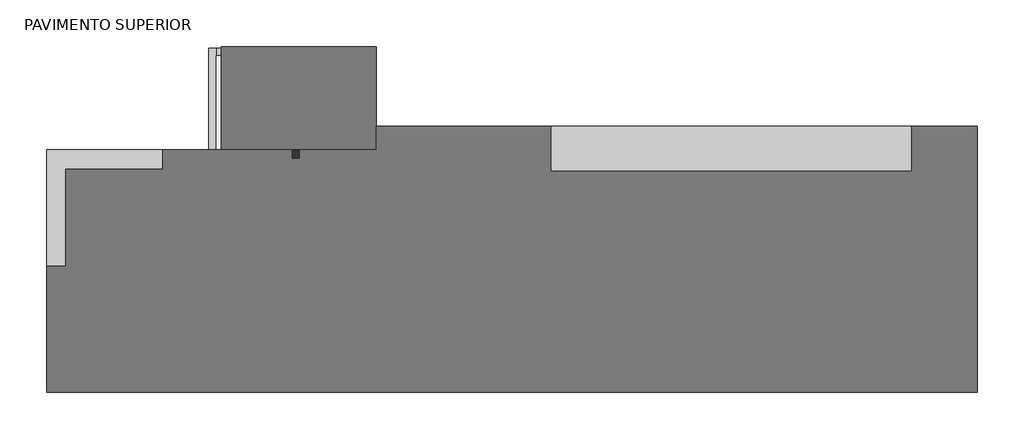
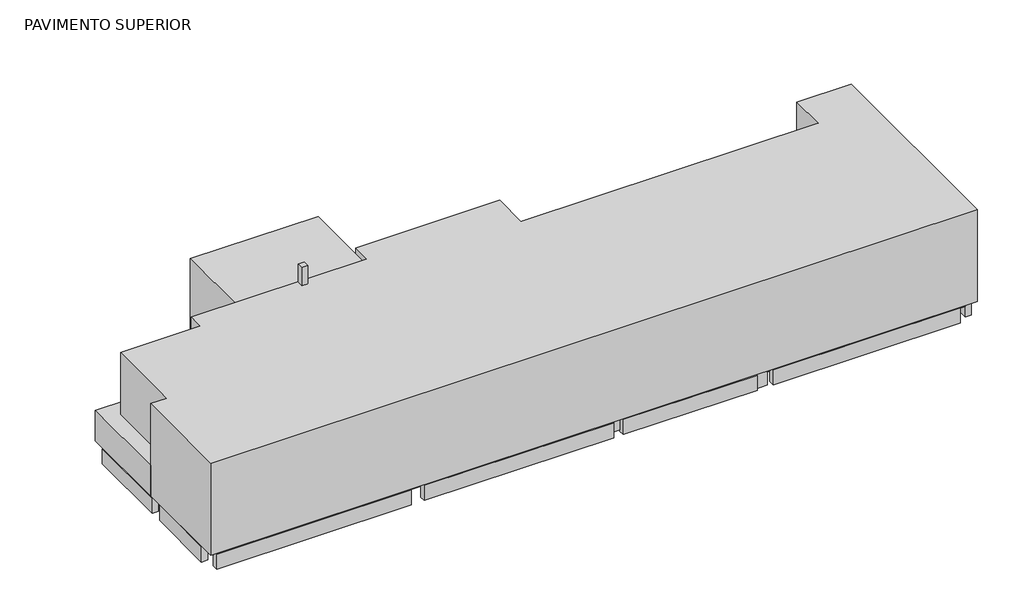
# One storey: 21 beams, 14 slabs, 2 proxies, 1 column.
# Revit data of these elements (continued)
# Element 11 (IfcBeam, "TQS - Viga retangular : 19.0 x 50.0") (continued)
#   Resultado de Ensaios fck (MPa) = 0
#   Unique TQS ID = -269
#   Principal = yes
#   Structural Material = none
#   Phase Created = CC_AP/ESTR
# Element 12 (IfcBeam, "TQS - Viga retangular : 19.0 x 50.0")
#   Uso = "ESTRUTURA"
#   Titulo = "V212"
#   Chave = "-271"
#   Tipo Elemento = "Viga"
#   SHA1 = "8138B3183DD0AFA166592BC9D25644F30CE3F0DB"
#   Revisão = ""
#   Tipo de carga = ""
#   Divisor de flexao = ""
#   Secao = ""
#   Configuracao = ""
#   Angulo (graus) = ""
#   Detalhamento = ""
#   Casos de vento manual = ""
#   Tipo = ""
#   Alcas = ""
#   Furos = ""
#   Pino = ""
#   Distribuicao = ""
#   Solidarizado = ""
#   Solidarizar na montagem = ""
#   Unir com o próximo = ""
#   Grupo pre moldado = ""
#   Verificado = ""
#   Concreto C = ""
#   Taxa de armadura (kgf/m³) = 0
#   Carga (tf/m²) = 0
#   Carga (tf/m) = 0
#   Carga (tf) = 0
#   Altura = 0.50 m
#   Rebaixo = 0.07 m
#   Largura = 0.19 m
#   Distancia a face = 0.00 m
#   Distancia ao eixo = 0.00 m
#   Altura gerber esquerda = 0.00 m
#   Largura gerber esquerda = 0.00 m
#   Altura gerber direita = 0.00 m
#   Largura gerber direita = 0.00 m
#   Resultado de Ensaios fck (MPa) = 0
#   Unique TQS ID = -271
#   Principal = yes
#   Structural Material = none
#   Phase Created = CC_AP/ESTR
# Element 13 (IfcBeam, "TQS - Viga retangular : 19.0 x 50.0")
#   Uso = "ESTRUTURA"
#   Titulo = "V204"
#   Chave = "-275"
#   Tipo Elemento = "Viga"
#   SHA1 = "02E3894711F00981ED511C33D176E4C517E4EA69"
#   Revisão = ""
#   Tipo de carga = ""
#   Divisor de flexao = ""
#   Secao = ""
#   Configuracao = ""
#   Angulo (graus) = ""
#   Detalhamento = ""
#   Casos de vento manual = ""
#   Tipo = ""
#   Alcas = ""
#   Furos = ""
#   Pino = ""
#   Distribuicao = ""
#   Solidarizado = ""
#   Solidarizar na montagem = ""
#   Unir com o próximo = ""
#   Grupo pre moldado = ""
#   Verificado = ""
#   Concreto C = ""
#   Taxa de armadura (kgf/m³) = 0
#   Carga (tf/m²) = 0
#   Carga (tf/m) = 0
#   Carga (tf) = 0
#   Altura = 0.50 m
#   Rebaixo = 0.07 m
#   Largura = 0.19 m
#   Distancia a face = 0.00 m
#   Distancia ao eixo = 0.00 m
#   Altura gerber esquerda = 0.00 m
#   Largura gerber esquerda = 0.00 m
#   Altura gerber direita = 0.00 m
#   Largura gerber direita = 0.00 m
#   Resultado de Ensaios fck (MPa) = 0
#   Unique TQS ID = -275
#   Principal = yes
#   Structural Material = none
#   Phase Created = CC_AP/ESTR
# Element 14 (IfcBeam, "TQS - Viga retangular : 19.0 x 50.0")
#   Uso = "ESTRUTURA"
#   Titulo = "V220"
#   Chave = "-277"
#   Tipo Elemento = "Viga"
#   SHA1 = "53FFBE44C6DCAED37B6C8CE186A7B735EF97D81B"
#   Revisão = ""
#   Tipo de carga = ""
#   Divisor de flexao = ""
#   Secao = ""
#   Configuracao = ""
#   Angulo (graus) = ""
#   Detalhamento = ""
#   Casos de vento manual = ""
#   Tipo = ""
#   Alcas = ""
#   Furos = ""
#   Pino = ""
#   Distribuicao = ""
#   Solidarizado = ""
#   Solidarizar na montagem = ""
#   Unir com o próximo = ""
#   Grupo pre moldado = ""
#   Verificado = ""
#   Concreto C = ""
#   Taxa de armadura (kgf/m³) = 0
#   Carga (tf/m²) = 0
#   Carga (tf/m) = 0
#   Carga (tf) = 0
#   Altura = 0.50 m
#   Rebaixo = 0.07 m
#   Largura = 0.19 m
#   Distancia a face = 0.00 m
#   Distancia ao eixo = 0.00 m
#   Altura gerber esquerda = 0.00 m
#   Largura gerber esquerda = 0.00 m
#   Altura gerber direita = 0.00 m
#   Largura gerber direita = 0.00 m
#   Resultado de Ensaios fck (MPa) = 0
#   Unique TQS ID = -277
#   Principal = yes
#   Structural Material = none
#   Phase Created = CC_AP/ESTR
# Element 15 (IfcBeam, "TQS - Viga retangular : 19.0 x 50.0")
#   Uso = "ESTRUTURA"
#   Titulo = "V205"
#   Chave = "-282"
#   Tipo Elemento = "Viga"
#   SHA1 = "42659F1FB713DA20C0E97ED290CCDAD82A2232BE"
#   Revisão = ""
#   Tipo de carga = ""
#   Divisor de flexao = ""
#   Secao = ""
#   Configuracao = ""
#   Angulo (graus) = ""
#   Detalhamento = ""
#   Casos de vento manual = ""
#   Tipo = ""
#   Alcas = ""
#   Furos = ""
#   Pino = ""
#   Distribuicao = ""
#   Solidarizado = ""
#   Solidarizar na montagem = ""
#   Unir com o próximo = ""
#   Grupo pre moldado = ""
#   Verificado = ""
#   Concreto C = ""
#   Taxa de armadura (kgf/m³) = 0
#   Carga (tf/m²) = 0
#   Carga (tf/m) = 0
#   Carga (tf) = 0
#   Altura = 0.50 m
#   Rebaixo = 0.07 m
#   Largura = 0.19 m
#   Distancia a face = 0.00 m
#   Distancia ao eixo = 0.00 m
#   Altura gerber esquerda = 0.00 m
#   Largura gerber esquerda = 0.00 m
#   Altura gerber direita = 0.00 m
#   Largura gerber direita = 0.00 m
#   Resultado de Ensaios fck (MPa) = 0
#   Unique TQS ID = -282
#   Principal = yes
#   Structural Material = none
#   Phase Created = CC_AP/ESTR
# Element 16 (IfcBeam, "TQS - Viga retangular : 19.0 x 50.0")
#   Uso = "ESTRUTURA"
#   Titulo = "V213"
#   Chave = "-292"
#   Tipo Elemento = "Viga"
#   SHA1 = "0FE3684D1E2234CA12F99F83675A4BD65DC506E8"
#   Revisão = ""
#   Tipo de carga = ""
#   Divisor de flexao = ""
#   Secao = ""
#   Configuracao = ""
#   Angulo (graus) = ""
#   Detalhamento = ""
#   Casos de vento manual = ""
#   Tipo = ""
#   Alcas = ""
#   Furos = ""
#   Pino = ""
#   Distribuicao = ""
#   Solidarizado = ""
#   Solidarizar na montagem = ""
#   Unir com o próximo = ""
#   Grupo pre moldado = ""
#   Verificado = ""
#   Concreto C = ""
#   Taxa de armadura (kgf/m³) = 0
#   Carga (tf/m²) = 0
#   Carga (tf/m) = 0
#   Carga (tf) = 0
#   Altura = 0.50 m
#   Rebaixo = 0.07 m
#   Largura = 0.19 m
#   Distancia a face = 0.00 m
#   Distancia ao eixo = 0.00 m
#   Altura gerber esquerda = 0.00 m
#   Largura gerber esquerda = 0.00 m
#   Altura gerber direita = 0.00 m
#   Largura gerber direita = 0.00 m
#   Resultado de Ensaios fck (MPa) = 0
#   Unique TQS ID = -292
#   Principal = yes
#   Structural Material = none
#   Phase Created = CC_AP/ESTR
# Element 17 (IfcBeam, "TQS - Viga retangular : 19.0 x 50.0")
#   Uso = "ESTRUTURA"
#   Titulo = "V216"
#   Chave = "-293"
#   Tipo Elemento = "Viga"
#   SHA1 = "A379C6197F25C7CB47ACBD41020AB1BAF3A8190D"
#   Revisão = ""
#   Tipo de carga = ""
#   Divisor de flexao = ""
#   Secao = ""
#   Configuracao = ""
#   Angulo (graus) = ""
#   Detalhamento = ""
#   Casos de vento manual = ""
#   Tipo = ""
#   Alcas = ""
#   Furos = ""
#   Pino = ""
#   Distribuicao = ""
#   Solidarizado = ""
#   Solidarizar na montagem = ""
#   Unir com o próximo = ""
#   Grupo pre moldado = ""
#   Verificado = ""
#   Concreto C = ""
#   Taxa de armadura (kgf/m³) = 0
#   Carga (tf/m²) = 0
#   Carga (tf/m) = 0
#   Carga (tf) = 0
#   Altura = 0.50 m
#   Rebaixo = 0.07 m
#   Largura = 0.19 m
#   Distancia a face = 0.00 m
#   Distancia ao eixo = 0.00 m
#   Altura gerber esquerda = 0.00 m
#   Largura gerber esquerda = 0.00 m
#   Altura gerber direita = 0.00 m
#   Largura gerber direita = 0.00 m
#   Resultado de Ensaios fck (MPa) = 0
#   Unique TQS ID = -293
#   Principal = yes
#   Structural Material = none
#   Phase Created = CC_AP/ESTR
# Element 18 (IfcBeam, "TQS - Viga retangular : 19.0 x 50.0")
#   Uso = "ESTRUTURA"
#   Titulo = "V201"
#   Chave = "-294"
#   Tipo Elemento = "Viga"
#   SHA1 = "3FA94C587EE4F3BD96CF329630B49136817C541B"
#   Revisão = ""
#   Tipo de carga = ""
#   Divisor de flexao = ""
#   Secao = ""
#   Configuracao = ""
#   Angulo (graus) = ""
#   Detalhamento = ""
#   Casos de vento manual = ""
#   Tipo = ""
#   Alcas = ""
#   Furos = ""
#   Pino = ""
#   Distribuicao = ""
#   Solidarizado = ""
#   Solidarizar na montagem = ""
#   Unir com o próximo = ""
#   Grupo pre moldado = ""
#   Verificado = ""
#   Concreto C = ""
#   Taxa de armadura (kgf/m³) = 0
#   Carga (tf/m²) = 0
#   Carga (tf/m) = 0
#   Carga (tf) = 0
#   Altura = 0.50 m
#   Rebaixo = 0.07 m
#   Largura = 0.19 m
#   Distancia a face = 0.00 m
#   Distancia ao eixo = 0.00 m
#   Altura gerber esquerda = 0.00 m
#   Largura gerber esquerda = 0.00 m
#   Altura gerber direita = 0.00 m
#   Largura gerber direita = 0.00 m
#   Resultado de Ensaios fck (MPa) = 0
#   Unique TQS ID = -294
#   Principal = yes
#   Structural Material = none
#   Phase Created = CC_AP/ESTR
# Element 19 (IfcBeam, "TQS - Viga retangular : 19.0 x 50.0")
#   Uso = "ESTRUTURA"
#   Titulo = "V203"
#   Chave = "-1337"
#   Tipo Elemento = "Viga"
#   SHA1 = "F25A04961C3A0A77CFDF86D87ECBEE6AEAF2B145"
#   Revisão = ""
#   Tipo de carga = ""
#   Divisor de flexao = ""
#   Secao = ""
#   Configuracao = ""
#   Angulo (graus) = ""
#   Detalhamento = ""
#   Casos de vento manual = ""
#   Tipo = ""
#   Alcas = ""
#   Furos = ""
#   Pino = ""
#   Distribuicao = ""
#   Solidarizado = ""
#   Solidarizar na montagem = ""
#   Unir com o próximo = ""
#   Grupo pre moldado = ""
#   Verificado = ""
#   Concreto C = ""
#   Taxa de armadura (kgf/m³) = 0
#   Carga (tf/m²) = 0
#   Carga (tf/m) = 0
#   Carga (tf) = 0
#   Altura = 0.50 m
#   Rebaixo = 0.07 m
#   Largura = 0.19 m
#   Distancia a face = 0.00 m
#   Distancia ao eixo = 0.00 m
#   Altura gerber esquerda = 0.00 m
#   Largura gerber esquerda = 0.00 m
#   Altura gerber direita = 0.00 m
#   Largura gerber direita = 0.00 m
#   Resultado de Ensaios fck (MPa) = 0
#   Unique TQS ID = -1337
#   Principal = yes
#   Structural Material = none
#   Phase Created = CC_AP/ESTR
# Element 20 (IfcBeam, "TQS - Viga retangular : 35.0 x 50.0")
#   Uso = "ESTRUTURA"
#   Titulo = "V218"
#   Chave = "-1330"
#   Tipo Elemento = "Viga"
#   SHA1 = "DF59D9C5ECE1DAFADA315DD633BF351C28CD7B23"
#   Revisão = ""
#   Tipo de carga = ""
#   Divisor de flexao = ""
#   Secao = ""
#   Configuracao = ""
#   Angulo (graus) = ""
#   Detalhamento = ""
#   Casos de vento manual = ""
#   Tipo = ""
#   Alcas = ""
#   Furos = ""
#   Pino = ""
#   Distribuicao = ""
#   Solidarizado = ""
#   Solidarizar na montagem = ""
#   Unir com o próximo = ""
#   Grupo pre moldado = ""
#   Verificado = ""
#   Concreto C = ""
#   Taxa de armadura (kgf/m³) = 0
#   Carga (tf/m²) = 0
#   Carga (tf/m) = 0
#   Carga (tf) = 0
#   Altura = 0.50 m
#   Rebaixo = 0.16 m
#   Largura = 0.35 m
#   Distancia a face = 0.00 m
#   Distancia ao eixo = 0.00 m
#   Altura gerber esquerda = 0.00 m
#   Largura gerber esquerda = 0.00 m
#   Altura gerber direita = 0.00 m
#   Largura gerber direita = 0.00 m
#   Resultado de Ensaios fck (MPa) = 0
#   Unique TQS ID = -1330
#   Principal = yes
#   Structural Material = none
#   Phase Created = CC_AP/ESTR
# Element 21 (IfcBeam, "TQS - Viga retangular : 35.0 x 59.0")
#   Uso = "ESTRUTURA"
#   Titulo = "V218"
#   Chave = "-1329"
#   Tipo Elemento = "Viga"
#   SHA1 = "67D04BBC0D1EFB8924A6F9E6F0DB65A2FA8FB170"
#   Revisão = ""
#   Tipo de carga = ""
#   Divisor de flexao = ""
#   Secao = ""
#   Configuracao = ""
#   Angulo (graus) = ""
#   Detalhamento = ""
#   Casos de vento manual = ""
#   Tipo = ""
#   Alcas = ""
#   Furos = ""
#   Pino = ""
#   Distribuicao = ""
#   Solidarizado = ""
#   Solidarizar na montagem = ""
#   Unir com o próximo = ""
#   Grupo pre moldado = ""
#   Verificado = ""
#   Concreto C = ""
#   Taxa de armadura (kgf/m³) = 0
#   Carga (tf/m²) = 0
#   Carga (tf/m) = 0
#   Carga (tf) = 0
#   Altura = 0.59 m
#   Rebaixo = 0.07 m
#   Largura = 0.35 m
#   Distancia a face = 0.00 m
#   Distancia ao eixo = 0.00 m
#   Altura gerber esquerda = 0.00 m
#   Largura gerber esquerda = 0.00 m
#   Altura gerber direita = 0.00 m
#   Largura gerber direita = 0.00 m
#   Resultado de Ensaios fck (MPa) = 0
#   Unique TQS ID = -1329
#   Principal = yes
#   Structural Material = none
#   Phase Created = CC_AP/ESTR
# Element 22 (IfcBuildingElementProxy, "SUÍTES E SALA ÍNTIMA : SUÍTES E SALA ÍNTIMA")
#   Phase Created = CC_EV
#   Materials on its faces: "Forma padrão"
# Element 23 (IfcBuildingElementProxy, "TERRAÇO : TERRAÇO")
#   Phase Created = CC_EV
#   Materials on its faces: "Forma padrão"
# Element 24 (IfcColumn, "TQS - Pilar retangular : 19.0 x 19.0")
#   Uso = "ESTRUTURA"
#   Titulo = "P17.2"
#   Chave = "P17.2//0"
#   Tipo Elemento = "Pilar"
#   SHA1 = "5EAE41CEDCF7AC730D71745C540256BEBFE0F897"
#   Revisão = ""
#   Tipo de carga = ""
#   Divisor de flexao = ""
#   Secao = "R 19/19 180°"
#   Configuracao = ""
#   Angulo (graus) = ""
#   Detalhamento = ""
#   Casos de vento manual = ""
#   Tipo = ""
#   Alcas = ""
#   Furos = ""
#   Pino = ""
#   Distribuicao = ""
#   Solidarizado = ""
#   Solidarizar na montagem = ""
#   Unir com o próximo = ""
#   Grupo pre moldado = ""
#   Verificado = ""
#   Concreto C = ""
#   Taxa de armadura (kgf/m³) = 0
#   Carga (tf/m²) = 0
#   Carga (tf/m) = 0
#   Carga (tf) = 0
#   Altura = 3.05 m
#   Rebaixo = 0.00 m
#   Altura da fundacao = 0.00 m
#   Largura = 0.00 m
#   Distancia a face = 0.00 m
#   Distancia ao eixo = 0.00 m
#   Resultado de Ensaios fck (MPa) = 0
#   Unique TQS ID = -1881
#   Principal = yes
#   Nasce = yes
#   Morre = yes
#   Cabeca de Pilar = no
#   Structural Material = Concrete - Cast-in-Place Concrete
#   Phase Created = CC_AP/ESTR
#   Materials on its faces: "Concrete - Cast-in-Place Concrete"
# Element 25 (IfcSlab, "TQS h=15")
#   Uso = "ESTRUTURA"
#   Titulo = "L2"
#   Chave = "-293"
#   Tipo Elemento = "Laje"
#   SHA1 = "30CE78691B5EE77FC65FFF8CB4530939F77CBC39"
#   Revisão = ""
#   Tipo de carga = ""
#   Divisor de flexao = ""
#   Fabricante = ""
#   Enchimento = ""
#   Mini painel = ""
#   Blocos por nervura = ""
#   Secao = ""
#   Configuracao = ""
#   Angulo (graus) = "0"
#   Detalhamento = ""
#   Casos de vento manual = ""
#   Tipo = "Pré-moldada"
#   Alcas = ""
#   Furos = ""
#   Pino = ""
#   Distribuicao = ""
#   Solidarizado = ""
#   Solidarizar na montagem = ""
#   Unir com o próximo = ""
#   Grupo pre moldado = ""
#   Verificado = ""
#   Concreto C = ""
#   Height Offset From Level = -0.07 m
#   Taxa de armadura (kgf/m³) = 0
#   Carga (tf/m²) = 0
#   Carga (tf/m) = 0
#   Carga (tf) = 0
#   Altura = 0.15 m
#   Capa = 0.04 m
#   Capa inferior = 0.00 m
#   Altura da nervura = 0.11 m
#   Enchimento (tf/m³) = 0.02
#   Largura inferior X = 0.00 m
#   Distancia inferior X = 0.00 m
#   Largura inferior Y = 0.00 m
#   Distancia inferior Y = 0.00 m
#   Largura vigota = 0.00 m
#   Altura vigota = 0.00 m
#   Largura perfil = 0.00 m
#   Largura aba = 0.00 m
#   Altura perfil = 0.00 m
#   Nervura secundaria = 0.00 m
#   Desconto nervura secundaria = 0.00 m
#   Rebaixo = -0.07 m
#   Largura = 0.00 m
#   Distancia a face = 0.00 m
#   Distancia ao eixo = 0.00 m
#   Resultado de Ensaios fck (MPa) = 0
#   built-in parameter 1001954 = 1
#   Unique TQS ID = -293
#   Principal = yes
#   Phase Created = CC_AP/ESTR
#   Materials on its faces: ".MATERIAL GENÉRICO LAJE E PISO"
# Element 26 (IfcSlab, "TQS h=15")
#   Uso = "ESTRUTURA"
#   Titulo = "L8"
#   Chave = "-294"
#   Tipo Elemento = "Laje"
#   SHA1 = "A0E1DD69F653FC0ADE227BB067D3F3136C230378"
#   Revisão = ""
#   Tipo de carga = ""
#   Divisor de flexao = ""
#   Fabricante = ""
#   Enchimento = ""
#   Mini painel = ""
#   Blocos por nervura = ""
#   Secao = ""
#   Configuracao = ""
#   Angulo (graus) = "0"
#   Detalhamento = ""
#   Casos de vento manual = ""
#   Tipo = "Pré-moldada"
#   Alcas = ""
#   Furos = ""
#   Pino = ""
#   Distribuicao = ""
#   Solidarizado = ""
#   Solidarizar na montagem = ""
#   Unir com o próximo = ""
#   Grupo pre moldado = ""
#   Verificado = ""
#   Concreto C = ""
#   Height Offset From Level = -0.07 m
#   Taxa de armadura (kgf/m³) = 0
#   Carga (tf/m²) = 0
#   Carga (tf/m) = 0
#   Carga (tf) = 0
#   Altura = 0.15 m
#   Capa = 0.04 m
#   Capa inferior = 0.00 m
#   Altura da nervura = 0.11 m
#   Enchimento (tf/m³) = 0.02
#   Largura inferior X = 0.00 m
#   Distancia inferior X = 0.00 m
#   Largura inferior Y = 0.00 m
#   Distancia inferior Y = 0.00 m
#   Largura vigota = 0.00 m
#   Altura vigota = 0.00 m
#   Largura perfil = 0.00 m
#   Largura aba = 0.00 m
#   Altura perfil = 0.00 m
#   Nervura secundaria = 0.00 m
#   Desconto nervura secundaria = 0.00 m
#   Rebaixo = -0.07 m
#   Largura = 0.00 m
#   Distancia a face = 0.00 m
#   Distancia ao eixo = 0.00 m
#   Resultado de Ensaios fck (MPa) = 0
#   built-in parameter 1001954 = 1
#   Unique TQS ID = -294
#   Principal = yes
#   Phase Created = CC_AP/ESTR
#   Materials on its faces: ".MATERIAL GENÉRICO LAJE E PISO"
# Element 27 (IfcSlab, "TQS h=15")
#   Uso = "ESTRUTURA"
#   Titulo = "L12"
#   Chave = "-1341"
#   Tipo Elemento = "Laje"
#   SHA1 = "62DBD7FB482137E78B4EBE55A5ED8AF7F76A63B1"
#   Revisão = ""
#   Tipo de carga = ""
#   Divisor de flexao = ""
#   Fabricante = ""
#   Enchimento = ""
#   Mini painel = ""
#   Blocos por nervura = ""
#   Secao = ""
#   Configuracao = ""
#   Angulo (graus) = "90"
#   Detalhamento = ""
#   Casos de vento manual = ""
#   Tipo = "Pré-moldada"
#   Alcas = ""
#   Furos = ""
#   Pino = ""
#   Distribuicao = ""
#   Solidarizado = ""
#   Solidarizar na montagem = ""
#   Unir com o próximo = ""
#   Grupo pre moldado = ""
#   Verificado = ""
#   Concreto C = ""
#   Height Offset From Level = -0.07 m
#   Taxa de armadura (kgf/m³) = 0
#   Carga (tf/m²) = 0
#   Carga (tf/m) = 0
#   Carga (tf) = 0
#   Altura = 0.15 m
#   Capa = 0.04 m
#   Capa inferior = 0.00 m
#   Altura da nervura = 0.11 m
#   Enchimento (tf/m³) = 0.02
#   Largura inferior X = 0.00 m
#   Distancia inferior X = 0.00 m
#   Largura inferior Y = 0.00 m
#   Distancia inferior Y = 0.00 m
#   Largura vigota = 0.00 m
#   Altura vigota = 0.00 m
#   Largura perfil = 0.00 m
#   Largura aba = 0.00 m
#   Altura perfil = 0.00 m
#   Nervura secundaria = 0.00 m
#   Desconto nervura secundaria = 0.00 m
#   Rebaixo = -0.07 m
#   Largura = 0.00 m
#   Distancia a face = 0.00 m
#   Distancia ao eixo = 0.00 m
#   Resultado de Ensaios fck (MPa) = 0
#   built-in parameter 1001954 = 1
#   Unique TQS ID = -1341
#   Principal = yes
#   Phase Created = CC_AP/ESTR
#   Materials on its faces: ".MATERIAL GENÉRICO LAJE E PISO"
# Element 28 (IfcSlab, "TQS h=15")
#   Uso = "ESTRUTURA"
#   Titulo = "L7"
#   Chave = "-289"
#   Tipo Elemento = "Laje"
#   SHA1 = "00FB641EB890BE101A5F35BC568EFA8C03036441"
#   Revisão = ""
#   Tipo de carga = ""
#   Divisor de flexao = ""
#   Fabricante = ""
#   Enchimento = ""
#   Mini painel = ""
#   Blocos por nervura = ""
#   Secao = ""
#   Configuracao = ""
#   Angulo (graus) = "90"
#   Detalhamento = ""
#   Casos de vento manual = ""
#   Tipo = "Pré-moldada"
#   Alcas = ""
#   Furos = ""
#   Pino = ""
#   Distribuicao = ""
#   Solidarizado = ""
#   Solidarizar na montagem = ""
#   Unir com o próximo = ""
#   Grupo pre moldado = ""
#   Verificado = ""
#   Concreto C = ""
#   Height Offset From Level = -0.07 m
#   Taxa de armadura (kgf/m³) = 0
#   Carga (tf/m²) = 0
#   Carga (tf/m) = 0
#   Carga (tf) = 0
#   Altura = 0.15 m
#   Capa = 0.04 m
#   Capa inferior = 0.00 m
#   Altura da nervura = 0.11 m
#   Enchimento (tf/m³) = 0.02
#   Largura inferior X = 0.00 m
#   Distancia inferior X = 0.00 m
#   Largura inferior Y = 0.00 m
#   Distancia inferior Y = 0.00 m
#   Largura vigota = 0.00 m
#   Altura vigota = 0.00 m
#   Largura perfil = 0.00 m
#   Largura aba = 0.00 m
#   Altura perfil = 0.00 m
#   Nervura secundaria = 0.00 m
#   Desconto nervura secundaria = 0.00 m
#   Rebaixo = -0.07 m
#   Largura = 0.00 m
#   Distancia a face = 0.00 m
#   Distancia ao eixo = 0.00 m
#   Resultado de Ensaios fck (MPa) = 0
#   built-in parameter 1001954 = 1
#   Unique TQS ID = -289
#   Principal = yes
#   Phase Created = CC_AP/ESTR
#   Materials on its faces: ".MATERIAL GENÉRICO LAJE E PISO"
# Element 29 (IfcSlab, "TQS h=15")
#   Uso = "ESTRUTURA"
#   Titulo = "L3"
#   Chave = "-290"
#   Tipo Elemento = "Laje"
#   SHA1 = "5CC856C49E54B4625D4D3CA5C635EB29D7F82A16"
#   Revisão = ""
#   Tipo de carga = ""
#   Divisor de flexao = ""
#   Fabricante = ""
#   Enchimento = ""
#   Mini painel = ""
#   Blocos por nervura = ""
#   Secao = ""
#   Configuracao = ""
#   Angulo (graus) = "90"
#   Detalhamento = ""
#   Casos de vento manual = ""
#   Tipo = "Pré-moldada"
#   Alcas = ""
#   Furos = ""
#   Pino = ""
#   Distribuicao = ""
#   Solidarizado = ""
#   Solidarizar na montagem = ""
#   Unir com o próximo = ""
#   Grupo pre moldado = ""
#   Verificado = ""
#   Concreto C = ""
#   Height Offset From Level = -0.07 m
#   Taxa de armadura (kgf/m³) = 0
#   Carga (tf/m²) = 0
#   Carga (tf/m) = 0
#   Carga (tf) = 0
#   Altura = 0.15 m
#   Capa = 0.04 m
#   Capa inferior = 0.00 m
#   Altura da nervura = 0.11 m
#   Enchimento (tf/m³) = 0.02
#   Largura inferior X = 0.00 m
#   Distancia inferior X = 0.00 m
#   Largura inferior Y = 0.00 m
#   Distancia inferior Y = 0.00 m
#   Largura vigota = 0.00 m
#   Altura vigota = 0.00 m
#   Largura perfil = 0.00 m
#   Largura aba = 0.00 m
#   Altura perfil = 0.00 m
#   Nervura secundaria = 0.00 m
#   Desconto nervura secundaria = 0.00 m
#   Rebaixo = -0.07 m
#   Largura = 0.00 m
#   Distancia a face = 0.00 m
#   Distancia ao eixo = 0.00 m
#   Resultado de Ensaios fck (MPa) = 0
#   built-in parameter 1001954 = 1
#   Unique TQS ID = -290
#   Principal = yes
#   Phase Created = CC_AP/ESTR
#   Materials on its faces: ".MATERIAL GENÉRICO LAJE E PISO"
# Element 30 (IfcSlab, "TQS h=15")
#   Uso = "ESTRUTURA"
#   Titulo = "L4"
#   Chave = "-291"
#   Tipo Elemento = "Laje"
#   SHA1 = "E1E752CC52417E869C2ECB3AAEF17918D9AB4584"
#   Revisão = ""
#   Tipo de carga = ""
#   Divisor de flexao = ""
#   Fabricante = ""
#   Enchimento = ""
#   Mini painel = ""
#   Blocos por nervura = ""
#   Secao = ""
#   Configuracao = ""
#   Angulo (graus) = "90"
#   Detalhamento = ""
#   Casos de vento manual = ""
#   Tipo = "Pré-moldada"
#   Alcas = ""
#   Furos = ""
#   Pino = ""
#   Distribuicao = ""
#   Solidarizado = ""
#   Solidarizar na montagem = ""
#   Unir com o próximo = ""
#   Grupo pre moldado = ""
#   Verificado = ""
#   Concreto C = ""
#   Height Offset From Level = -0.07 m
#   Taxa de armadura (kgf/m³) = 0
#   Carga (tf/m²) = 0
#   Carga (tf/m) = 0
#   Carga (tf) = 0
#   Altura = 0.15 m
#   Capa = 0.04 m
#   Capa inferior = 0.00 m
#   Altura da nervura = 0.11 m
#   Enchimento (tf/m³) = 0.02
#   Largura inferior X = 0.00 m
#   Distancia inferior X = 0.00 m
#   Largura inferior Y = 0.00 m
#   Distancia inferior Y = 0.00 m
#   Largura vigota = 0.00 m
#   Altura vigota = 0.00 m
#   Largura perfil = 0.00 m
#   Largura aba = 0.00 m
#   Altura perfil = 0.00 m
#   Nervura secundaria = 0.00 m
#   Desconto nervura secundaria = 0.00 m
#   Rebaixo = -0.07 m
#   Largura = 0.00 m
#   Distancia a face = 0.00 m
#   Distancia ao eixo = 0.00 m
#   Resultado de Ensaios fck (MPa) = 0
#   built-in parameter 1001954 = 1
#   Unique TQS ID = -291
#   Principal = yes
#   Phase Created = CC_AP/ESTR
#   Materials on its faces: ".MATERIAL GENÉRICO LAJE E PISO"
# Element 31 (IfcSlab, "TQS h=15")
#   Uso = "ESTRUTURA"
#   Titulo = "L1"
#   Chave = "-782"
#   Tipo Elemento = "Laje"
#   SHA1 = "243054E1496AE50C7A59F49C35E9A6C4CBFBF802"
#   Revisão = ""
#   Tipo de carga = ""
#   Divisor de flexao = ""
#   Fabricante = ""
#   Enchimento = ""
#   Mini painel = ""
#   Blocos por nervura = ""
#   Secao = ""
#   Configuracao = ""
#   Angulo (graus) = "0"
#   Detalhamento = ""
#   Casos de vento manual = ""
#   Tipo = "Pré-moldada"
#   Alcas = ""
#   Furos = ""
#   Pino = ""
#   Distribuicao = ""
#   Solidarizado = ""
#   Solidarizar na montagem = ""
#   Unir com o próximo = ""
#   Grupo pre moldado = ""
#   Verificado = ""
#   Concreto C = ""
#   Height Offset From Level = -0.07 m
#   Taxa de armadura (kgf/m³) = 0
#   Carga (tf/m²) = 0
#   Carga (tf/m) = 0
#   Carga (tf) = 0
#   Altura = 0.15 m
#   Capa = 0.04 m
#   Capa inferior = 0.00 m
#   Altura da nervura = 0.11 m
#   Enchimento (tf/m³) = 0.02
#   Largura inferior X = 0.00 m
#   Distancia inferior X = 0.00 m
#   Largura inferior Y = 0.00 m
#   Distancia inferior Y = 0.00 m
#   Largura vigota = 0.00 m
#   Altura vigota = 0.00 m
#   Largura perfil = 0.00 m
#   Largura aba = 0.00 m
#   Altura perfil = 0.00 m
#   Nervura secundaria = 0.00 m
#   Desconto nervura secundaria = 0.00 m
#   Rebaixo = -0.07 m
#   Largura = 0.00 m
#   Distancia a face = 0.00 m
#   Distancia ao eixo = 0.00 m
#   Resultado de Ensaios fck (MPa) = 0
#   built-in parameter 1001954 = 1
#   Unique TQS ID = -782
#   Principal = yes
#   Phase Created = CC_AP/ESTR
#   Materials on its faces: ".MATERIAL GENÉRICO LAJE E PISO"
# Element 32 (IfcSlab, "TQS h=15")
#   Uso = "ESTRUTURA"
#   Titulo = "L5"
#   Chave = "-324"
#   Tipo Elemento = "Laje"
#   SHA1 = "6BEC4C6D90655AA68C15FC8554BD79BC3B34892D"
#   Revisão = ""
#   Tipo de carga = ""
#   Divisor de flexao = ""
#   Fabricante = ""
#   Enchimento = ""
#   Mini painel = ""
#   Blocos por nervura = ""
#   Secao = ""
#   Configuracao = ""
#   Angulo (graus) = "0"
#   Detalhamento = ""
#   Casos de vento manual = ""
#   Tipo = "Maciça"
#   Alcas = ""
#   Furos = ""
#   Pino = ""
#   Distribuicao = ""
#   Solidarizado = ""
#   Solidarizar na montagem = ""
#   Unir com o próximo = ""
#   Grupo pre moldado = ""
#   Verificado = ""
#   Concreto C = ""
#   Height Offset From Level = -0.07 m
#   Taxa de armadura (kgf/m³) = 0
#   Carga (tf/m²) = 0
#   Carga (tf/m) = 0
#   Carga (tf) = 0
#   Altura = 0.15 m
#   Capa = 0.00 m
#   Capa inferior = 0.00 m
#   Altura da nervura = 0.00 m
#   Enchimento (tf/m³) = 0
#   Largura inferior X = 0.00 m
#   Distancia inferior X = 0.00 m
#   Largura inferior Y = 0.00 m
#   Distancia inferior Y = 0.00 m
#   Largura vigota = 0.00 m
#   Altura vigota = 0.00 m
#   Largura perfil = 0.00 m
#   Largura aba = 0.00 m
#   Altura perfil = 0.00 m
#   Nervura secundaria = 0.00 m
#   Desconto nervura secundaria = 0.00 m
#   Rebaixo = -0.07 m
#   Largura = 0.00 m
#   Distancia a face = 0.00 m
#   Distancia ao eixo = 0.00 m
#   Resultado de Ensaios fck (MPa) = 0
#   built-in parameter 1001954 = 1
#   Unique TQS ID = -324
#   Principal = yes
#   Phase Created = CC_AP/ESTR
#   Materials on its faces: ".MATERIAL GENÉRICO LAJE E PISO"
# Element 33 (IfcSlab, "TQS h=15")
#   Uso = "ESTRUTURA"
#   Titulo = "L6"
#   Chave = "-325"
#   Tipo Elemento = "Laje"
#   SHA1 = "45A1BB14EB53BA680F766E33394AE66BA68CD49B"
#   Revisão = ""
#   Tipo de carga = ""
#   Divisor de flexao = ""
#   Fabricante = ""
#   Enchimento = ""
#   Mini painel = ""
#   Blocos por nervura = ""
#   Secao = ""
#   Configuracao = ""
#   Angulo (graus) = "0"
#   Detalhamento = ""
#   Casos de vento manual = ""
#   Tipo = "Maciça"
#   Alcas = ""
#   Furos = ""
#   Pino = ""
#   Distribuicao = ""
#   Solidarizado = ""
#   Solidarizar na montagem = ""
#   Unir com o próximo = ""
#   Grupo pre moldado = ""
#   Verificado = ""
#   Concreto C = ""
#   Height Offset From Level = -0.07 m
#   Taxa de armadura (kgf/m³) = 0
#   Carga (tf/m²) = 0
#   Carga (tf/m) = 0
#   Carga (tf) = 0
#   Altura = 0.15 m
#   Capa = 0.00 m
#   Capa inferior = 0.00 m
#   Altura da nervura = 0.00 m
#   Enchimento (tf/m³) = 0
#   Largura inferior X = 0.00 m
#   Distancia inferior X = 0.00 m
#   Largura inferior Y = 0.00 m
#   Distancia inferior Y = 0.00 m
#   Largura vigota = 0.00 m
#   Altura vigota = 0.00 m
#   Largura perfil = 0.00 m
#   Largura aba = 0.00 m
#   Altura perfil = 0.00 m
#   Nervura secundaria = 0.00 m
#   Desconto nervura secundaria = 0.00 m
#   Rebaixo = -0.07 m
#   Largura = 0.00 m
#   Distancia a face = 0.00 m
#   Distancia ao eixo = 0.00 m
#   Resultado de Ensaios fck (MPa) = 0
#   built-in parameter 1001954 = 1
#   Unique TQS ID = -325
#   Principal = yes
#   Phase Created = CC_AP/ESTR
#   Materials on its faces: ".MATERIAL GENÉRICO LAJE E PISO"
# Element 34 (IfcSlab, "TQS h=15")
#   Uso = "ESTRUTURA"
#   Titulo = "L10"
#   Chave = "-1358"
#   Tipo Elemento = "Laje"
#   SHA1 = "4893D49A38E51302E187866BCF6B5717B0F83667"
#   Revisão = ""
#   Tipo de carga = ""
#   Divisor de flexao = ""
#   Fabricante = ""
#   Enchimento = ""
#   Mini painel = ""
#   Blocos por nervura = ""
#   Secao = ""
#   Configuracao = ""
#   Angulo (graus) = "90"
#   Detalhamento = ""
#   Casos de vento manual = ""
#   Tipo = "Pré-moldada"
#   Alcas = ""
#   Furos = ""
#   Pino = ""
#   Distribuicao = ""
#   Solidarizado = ""
#   Solidarizar na montagem = ""
#   Unir com o próximo = ""
#   Grupo pre moldado = ""
#   Verificado = ""
#   Concreto C = ""
#   Height Offset From Level = -0.07 m
#   Taxa de armadura (kgf/m³) = 0
#   Carga (tf/m²) = 0
#   Carga (tf/m) = 0
#   Carga (tf) = 0
#   Altura = 0.15 m
#   Capa = 0.04 m
#   Capa inferior = 0.00 m
#   Altura da nervura = 0.11 m
#   Enchimento (tf/m³) = 0.02
#   Largura inferior X = 0.00 m
#   Distancia inferior X = 0.00 m
#   Largura inferior Y = 0.00 m
#   Distancia inferior Y = 0.00 m
#   Largura vigota = 0.00 m
#   Altura vigota = 0.00 m
#   Largura perfil = 0.00 m
#   Largura aba = 0.00 m
#   Altura perfil = 0.00 m
#   Nervura secundaria = 0.00 m
#   Desconto nervura secundaria = 0.00 m
#   Rebaixo = -0.07 m
#   Largura = 0.00 m
#   Distancia a face = 0.00 m
#   Distancia ao eixo = 0.00 m
#   Resultado de Ensaios fck (MPa) = 0
#   built-in parameter 1001954 = 1
#   Unique TQS ID = -1358
#   Principal = yes
#   Phase Created = CC_AP/ESTR
#   Materials on its faces: ".MATERIAL GENÉRICO LAJE E PISO"
# Element 35 (IfcSlab, "TQS h=15")
#   Uso = "ESTRUTURA"
#   Titulo = "L13"
#   Chave = "-1343"
#   Tipo Elemento = "Laje"
#   SHA1 = "8A662842B88D717936D380F689A228C2276122A1"
#   Revisão = ""
#   Tipo de carga = ""
#   Divisor de flexao = ""
#   Fabricante = ""
#   Enchimento = ""
#   Mini painel = ""
#   Blocos por nervura = ""
#   Secao = ""
#   Configuracao = ""
#   Angulo (graus) = "0"
#   Detalhamento = ""
#   Casos de vento manual = ""
#   Tipo = "Pré-moldada"
#   Alcas = ""
#   Furos = ""
#   Pino = ""
#   Distribuicao = ""
#   Solidarizado = ""
#   Solidarizar na montagem = ""
#   Unir com o próximo = ""
#   Grupo pre moldado = ""
#   Verificado = ""
#   Concreto C = ""
#   Height Offset From Level = -0.07 m
#   Taxa de armadura (kgf/m³) = 0
#   Carga (tf/m²) = 0
#   Carga (tf/m) = 0
#   Carga (tf) = 0
#   Altura = 0.15 m
#   Capa = 0.04 m
#   Capa inferior = 0.00 m
#   Altura da nervura = 0.11 m
#   Enchimento (tf/m³) = 0.02
#   Largura inferior X = 0.00 m
#   Distancia inferior X = 0.00 m
#   Largura inferior Y = 0.00 m
#   Distancia inferior Y = 0.00 m
#   Largura vigota = 0.00 m
#   Altura vigota = 0.00 m
#   Largura perfil = 0.00 m
#   Largura aba = 0.00 m
#   Altura perfil = 0.00 m
#   Nervura secundaria = 0.00 m
#   Desconto nervura secundaria = 0.00 m
#   Rebaixo = -0.07 m
#   Largura = 0.00 m
#   Distancia a face = 0.00 m
#   Distancia ao eixo = 0.00 m
#   Resultado de Ensaios fck (MPa) = 0
#   built-in parameter 1001954 = 1
#   Unique TQS ID = -1343
#   Principal = yes
#   Phase Created = CC_AP/ESTR
#   Materials on its faces: ".MATERIAL GENÉRICO LAJE E PISO"
# Element 36 (IfcSlab, "TQS h=15")
#   Uso = "ESTRUTURA"
#   Titulo = "L14"
#   Chave = "-1344"
#   Tipo Elemento = "Laje"
#   SHA1 = "E42E6546E86D746CC7E5C711CD7BCA8D3AB7D4E0"
#   Revisão = ""
#   Tipo de carga = ""
#   Divisor de flexao = ""
#   Fabricante = ""
#   Enchimento = ""
#   Mini painel = ""
#   Blocos por nervura = ""
#   Secao = ""
#   Configuracao = ""
#   Angulo (graus) = "0"
#   Detalhamento = ""
#   Casos de vento manual = ""
#   Tipo = "Pré-moldada"
#   Alcas = ""
#   Furos = ""
#   Pino = ""
#   Distribuicao = ""
#   Solidarizado = ""
#   Solidarizar na montagem = ""
#   Unir com o próximo = ""
#   Grupo pre moldado = ""
#   Verificado = ""
#   Concreto C = ""
#   Height Offset From Level = -0.07 m
#   Taxa de armadura (kgf/m³) = 0
#   Carga (tf/m²) = 0
#   Carga (tf/m) = 0
#   Carga (tf) = 0
#   Altura = 0.15 m
#   Capa = 0.04 m
#   Capa inferior = 0.00 m
#   Altura da nervura = 0.11 m
#   Enchimento (tf/m³) = 0.02
#   Largura inferior X = 0.00 m
#   Distancia inferior X = 0.00 m
#   Largura inferior Y = 0.00 m
#   Distancia inferior Y = 0.00 m
#   Largura vigota = 0.00 m
#   Altura vigota = 0.00 m
#   Largura perfil = 0.00 m
#   Largura aba = 0.00 m
#   Altura perfil = 0.00 m
#   Nervura secundaria = 0.00 m
#   Desconto nervura secundaria = 0.00 m
#   Rebaixo = -0.07 m
#   Largura = 0.00 m
#   Distancia a face = 0.00 m
#   Distancia ao eixo = 0.00 m
#   Resultado de Ensaios fck (MPa) = 0
#   built-in parameter 1001954 = 1
#   Unique TQS ID = -1344
#   Principal = yes
#   Phase Created = CC_AP/ESTR
#   Materials on its faces: ".MATERIAL GENÉRICO LAJE E PISO"
# Element 37 (IfcSlab, "TQS h=15")
#   Uso = "ESTRUTURA"
#   Titulo = "L9"
#   Chave = "-1359"
#   Tipo Elemento = "Laje"
#   SHA1 = "F01DC73605C6E75E49E3A1ECAE6F1D9103422308"
#   Revisão = ""
#   Tipo de carga = ""
#   Divisor de flexao = ""
#   Fabricante = ""
#   Enchimento = ""
#   Mini painel = ""
#   Blocos por nervura = ""
#   Secao = ""
#   Configuracao = ""
#   Angulo (graus) = "90"
#   Detalhamento = ""
#   Casos de vento manual = ""
#   Tipo = "Pré-moldada"
#   Alcas = ""
#   Furos = ""
#   Pino = ""
#   Distribuicao = ""
#   Solidarizado = ""
#   Solidarizar na montagem = ""
#   Unir com o próximo = ""
#   Grupo pre moldado = ""
#   Verificado = ""
#   Concreto C = ""
#   Height Offset From Level = -0.16 m
#   Taxa de armadura (kgf/m³) = 0
#   Carga (tf/m²) = 0
#   Carga (tf/m) = 0
#   Carga (tf) = 0
#   Altura = 0.15 m
#   Capa = 0.04 m
#   Capa inferior = 0.00 m
#   Altura da nervura = 0.11 m
#   Enchimento (tf/m³) = 0.02
#   Largura inferior X = 0.00 m
#   Distancia inferior X = 0.00 m
#   Largura inferior Y = 0.00 m
#   Distancia inferior Y = 0.00 m
#   Largura vigota = 0.00 m
#   Altura vigota = 0.00 m
#   Largura perfil = 0.00 m
#   Largura aba = 0.00 m
#   Altura perfil = 0.00 m
#   Nervura secundaria = 0.00 m
#   Desconto nervura secundaria = 0.00 m
#   Rebaixo = -0.16 m
#   Largura = 0.00 m
#   Distancia a face = 0.00 m
#   Distancia ao eixo = 0.00 m
#   Resultado de Ensaios fck (MPa) = 0
#   built-in parameter 1001954 = 1
#   Unique TQS ID = -1359
#   Principal = yes
#   Phase Created = CC_AP/ESTR
#   Materials on its faces: ".MATERIAL GENÉRICO LAJE E PISO"
# Element 38 (IfcSlab, "TQS h=15")
#   Uso = "ESTRUTURA"
#   Titulo = "L11"
#   Chave = "-1360"
#   Tipo Elemento = "Laje"
#   SHA1 = "DC277F3F4644E2283913F4010C0933E3E7135E2C"
#   Revisão = ""
#   Tipo de carga = ""
#   Divisor de flexao = ""
#   Fabricante = ""
#   Enchimento = ""
#   Mini painel = ""
#   Blocos por nervura = ""
#   Secao = ""
#   Configuracao = ""
#   Angulo (graus) = "90"
#   Detalhamento = ""
#   Casos de vento manual = ""
#   Tipo = "Pré-moldada"
#   Alcas = ""
#   Furos = ""
#   Pino = ""
#   Distribuicao = ""
#   Solidarizado = ""
#   Solidarizar na montagem = ""
#   Unir com o próximo = ""
#   Grupo pre moldado = ""
#   Verificado = ""
#   Concreto C = ""
#   Height Offset From Level = -0.16 m
#   Taxa de armadura (kgf/m³) = 0
#   Carga (tf/m²) = 0
#   Carga (tf/m) = 0
#   Carga (tf) = 0
#   Altura = 0.15 m
#   Capa = 0.04 m
#   Capa inferior = 0.00 m
#   Altura da nervura = 0.11 m
#   Enchimento (tf/m³) = 0.02
#   Largura inferior X = 0.00 m
#   Distancia inferior X = 0.00 m
#   Largura inferior Y = 0.00 m
#   Distancia inferior Y = 0.00 m
#   Largura vigota = 0.00 m
#   Altura vigota = 0.00 m
#   Largura perfil = 0.00 m
#   Largura aba = 0.00 m
#   Altura perfil = 0.00 m
#   Nervura secundaria = 0.00 m
#   Desconto nervura secundaria = 0.00 m
#   Rebaixo = -0.16 m
#   Largura = 0.00 m
#   Distancia a face = 0.00 m
#   Distancia ao eixo = 0.00 m
#   Resultado de Ensaios fck (MPa) = 0
#   built-in parameter 1001954 = 1
#   Unique TQS ID = -1360
#   Principal = yes
#   Phase Created = CC_AP/ESTR
#   Materials on its faces: ".MATERIAL GENÉRICO LAJE E PISO"
# Materials
#   "Concrete - Cast-in-Place Concrete": class "Unassigned", colour RGB 192 192 192, transparency 0
#   ".MATERIAL GENÉRICO LAJE E PISO": class ".CC_PAVIMENTAÇÃO", colour RGB 128 128 128, transparency 0, Description = "Material genérico para representação ND 200.", Cost = 0
#   "Forma padrão": class "Genérico", colour RGB 185 189 196, transparency 0.5, Cost = 0
